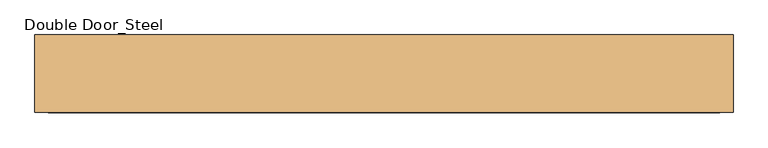
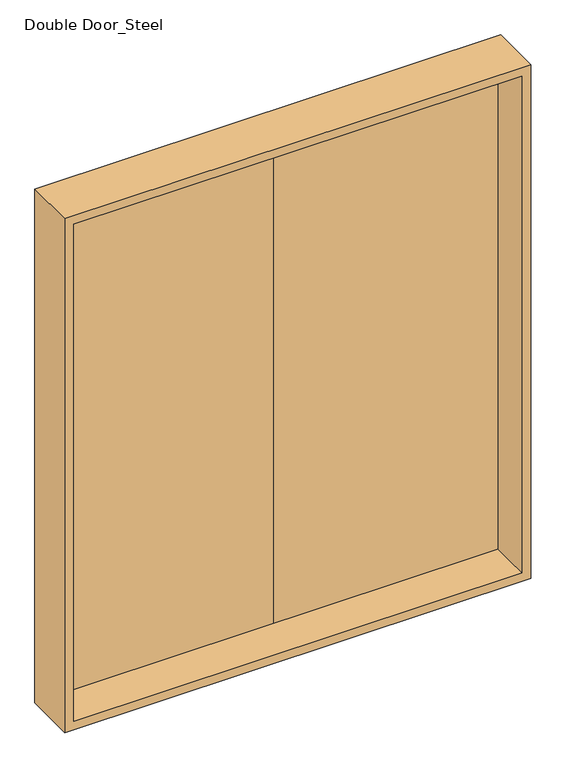
"""IFC4 building model written with IfcOpenShell, lengths in millimetres: door geometry, Double Door_Steel : H_DR_AR_B12_Double Door_Steel_W2000xH2100."""

import ifcopenshell
import ifcopenshell.guid

model = None  # the IFC model being written
_history = None  # IfcOwnerHistory: only IFC2X3 demands one
_inside = {}  # id of a spatial element -> (the spatial element, [elements in it])
_under = {}  # id of a project, library or spatial element -> (it, [spatial elements below it])
_declared = {}  # id of a project -> (the project, [libraries it declares])
_typed = {}  # id of a type object -> (the type object, [elements of that type])
_made_of = {}  # id of a material, layer set ... -> (it, [elements and type objects made of it])


def new_model(schema):
    """Start an empty IFC model of exactly this schema.

    Asked for "IFC4X3", IfcOpenShell would pick the latest addendum, in which some entities
    have other attributes; the version numbers below select the first issue.
    IFC2X3 requires an IfcOwnerHistory on every rooted entity: one is made here for all.
    """
    global model, _history
    if schema == "IFC4X3":
        model = ifcopenshell.file(schema_version=(4, 3, 0, 0))
    else:
        model = ifcopenshell.file(schema=schema)
    _inside.clear()
    _under.clear()
    _declared.clear()
    _typed.clear()
    _made_of.clear()
    _history = None
    if model.schema == "IFC2X3":
        org = make("IfcOrganization", Name="unknown")
        user = make(
            "IfcPersonAndOrganization",
            ThePerson=make("IfcPerson", FamilyName="unknown"),
            TheOrganization=org,
        )
        app = make(
            "IfcApplication",
            ApplicationDeveloper=org,
            Version="unknown",
            ApplicationFullName="unknown",
            ApplicationIdentifier="unknown",
        )
        _history = make(
            "IfcOwnerHistory",
            OwningUser=user,
            OwningApplication=app,
            ChangeAction="ADDED",
            CreationDate=0,
        )
    return model


def make(cls, **values):
    """One entity of the class cls with the attributes given. An attribute that is None is left unset."""
    return model.create_entity(
        cls, **{name: value for name, value in values.items() if value is not None}
    )


def rooted(cls, **values):
    """An entity with a GlobalId (a new one), such as an element, a storey or a relation."""
    return make(cls, GlobalId=ifcopenshell.guid.new(), OwnerHistory=_history, **values)


def si_unit(unit_type, name, prefix=None):
    """IfcSIUnit, for example si_unit("LENGTHUNIT", "METRE", prefix="MILLI")."""
    return make("IfcSIUnit", UnitType=unit_type, Prefix=prefix, Name=name)


def assignment(units):
    """IfcUnitAssignment: the units of a project."""
    return None if units is None else make("IfcUnitAssignment", Units=units)


def point(xyz):
    """IfcCartesianPoint."""
    return None if xyz is None else make("IfcCartesianPoint", Coordinates=xyz)


def direction(xyz):
    """IfcDirection."""
    return None if xyz is None else make("IfcDirection", DirectionRatios=xyz)


def frame(location, z_axis=None, x_axis=None):
    """IfcAxis2Placement3D, a coordinate frame: its origin and axes. An axis left out is left unset."""
    return make(
        "IfcAxis2Placement3D",
        Location=point(location),
        Axis=direction(z_axis),
        RefDirection=direction(x_axis),
    )


def origin():
    """The frame at (0, 0, 0) with its axes left unset."""
    return frame((0.0, 0.0, 0.0))


def place(relative_to, where):
    """IfcLocalPlacement: puts the frame where relative to a parent placement (None: the world)."""
    return make(
        "IfcLocalPlacement", PlacementRelTo=relative_to, RelativePlacement=where
    )


def context(
    kind, dimensions, precision=None, world=None, true_north=None, identifier=None
):
    """IfcGeometricRepresentationContext, for example the 3D "Model" context."""
    return make(
        "IfcGeometricRepresentationContext",
        ContextIdentifier=identifier,
        ContextType=kind,
        CoordinateSpaceDimension=dimensions,
        Precision=precision,
        WorldCoordinateSystem=world,
        TrueNorth=true_north,
    )


def project(units=None, contexts=None):
    """IfcProject with its units and contexts."""
    return rooted(
        "IfcProject",
        Name="project",
        RepresentationContexts=contexts,
        UnitsInContext=assignment(units),
    )


def spatial(cls, under=None, at=None, **own):
    """A site, building, storey or space (cls), placed at a placement, below another one or the project."""
    s = rooted(cls, ObjectPlacement=at, **own)
    if under is not None:
        _under.setdefault(under.id(), (under, []))[1].append(s)
    return s


def polyline(points):
    """IfcPolyline through the points."""
    return make("IfcPolyline", Points=[point(p) for p in points])


def outline(outer, holes=None, kind="AREA"):
    """IfcArbitraryClosedProfileDef: a profile drawn as a closed curve; with holes, ...WithVoids."""
    if holes is None:
        return make("IfcArbitraryClosedProfileDef", ProfileType=kind, OuterCurve=outer)
    return make(
        "IfcArbitraryProfileDefWithVoids",
        ProfileType=kind,
        OuterCurve=outer,
        InnerCurves=holes,
    )


def extrude(swept, where, along, depth):
    """IfcExtrudedAreaSolid: the profile swept, set in the frame where, extruded along a direction by depth."""
    return make(
        "IfcExtrudedAreaSolid",
        SweptArea=swept,
        Position=where,
        ExtrudedDirection=direction(along),
        Depth=depth,
    )


def faces_of(points, faces, orient=None, outer=None):
    """IfcFace entities. A face is a list of loops; a loop is a list of indices into points, from 0.

    orient and outer hold one flag for each loop. By default every Orientation is true, the
    first loop of a face is its IfcFaceOuterBound and the others are IfcFaceBound.
    """
    made = []
    for i, loops in enumerate(faces):
        bounds = []
        for j, loop in enumerate(loops):
            is_outer = j == 0 if outer is None else outer[i][j]
            bounds.append(
                make(
                    "IfcFaceOuterBound" if is_outer else "IfcFaceBound",
                    Bound=make("IfcPolyLoop", Polygon=[points[k] for k in loop]),
                    Orientation=True if orient is None else orient[i][j],
                )
            )
        made.append(make("IfcFace", Bounds=bounds))
    return made


def faceted_brep(points, faces, orient=None, outer=None, voids=None):
    """IfcFacetedBrep: a solid bounded by flat faces; with voids (closed shells), ...WithVoids."""
    shared = [point(p) for p in points]
    hull = make("IfcClosedShell", CfsFaces=faces_of(shared, faces, orient, outer))
    if voids is None:
        return make("IfcFacetedBrep", Outer=hull)
    return make(
        "IfcFacetedBrepWithVoids",
        Outer=hull,
        Voids=[
            make(cls, CfsFaces=faces_of(shared, fs, o, b)) for cls, fs, o, b in voids
        ],
    )


def shape(context_of_items, identifier, shape_type, items):
    """IfcShapeRepresentation: the items that make up one representation, for example the "Body"."""
    return make(
        "IfcShapeRepresentation",
        ContextOfItems=context_of_items,
        RepresentationIdentifier=identifier,
        RepresentationType=shape_type,
        Items=items,
    )


def source(mapping_origin, context_of_items, identifier, shape_type, items):
    """IfcRepresentationMap: a shape defined once, which mapped items show again and again."""
    return make(
        "IfcRepresentationMap",
        MappingOrigin=mapping_origin,
        MappedRepresentation=shape(context_of_items, identifier, shape_type, items),
    )


def transform(
    local_origin,
    x_axis=None,
    y_axis=None,
    z_axis=None,
    scale=None,
    scale2=None,
    scale3=None,
    uniform=True,
):
    """IfcCartesianTransformationOperator3D, or its non-uniform kind. x_axis, y_axis, z_axis: its Axis1, 2, 3."""
    if uniform:
        return make(
            "IfcCartesianTransformationOperator3D",
            Axis1=direction(x_axis),
            Axis2=direction(y_axis),
            LocalOrigin=point(local_origin),
            Scale=scale,
            Axis3=direction(z_axis),
        )
    return make(
        "IfcCartesianTransformationOperator3DnonUniform",
        Axis1=direction(x_axis),
        Axis2=direction(y_axis),
        LocalOrigin=point(local_origin),
        Scale=scale,
        Axis3=direction(z_axis),
        Scale2=scale2,
        Scale3=scale3,
    )


def mapped(mapping_source, mapping_target):
    """IfcMappedItem: shows the shape of a source again, moved by a transform."""
    return make(
        "IfcMappedItem", MappingSource=mapping_source, MappingTarget=mapping_target
    )


def made_of(thing, what):
    """Note that an element or type object is made of a material, layer set ...; save() writes the relation."""
    if what is not None:
        _made_of.setdefault(what.id(), (what, []))[1].append(thing)
    return thing


def element(
    cls,
    number,
    at=None,
    inside=None,
    cuts=None,
    type_object=None,
    material=None,
    context=None,
    identifier="Body",
    shape_type=None,
    held_by="IfcProductDefinitionShape",
    body=None,
    shapes=None,
    **own,
):
    """One element of the class cls, such as IfcWall. Its Tag is "e" and its number.

    at: its placement. inside: the storey or other place that contains it. cuts: it is an
    opening in that element (IfcRelVoidsElement). A single representation is given by context,
    identifier, shape_type and body (its items); several are given by shapes. held_by: the class
    of the entity that holds the representations. save() writes the other relations.
    """
    e = rooted(cls, Tag="e%d" % number, ObjectPlacement=at, **own)
    if body is not None:
        shapes = [shape(context, identifier, shape_type, body)]
    if shapes is not None:
        e.Representation = make(held_by, Representations=shapes)
    if inside is not None:
        _inside.setdefault(inside.id(), (inside, []))[1].append(e)
    if cuts is not None:
        rooted(
            "IfcRelVoidsElement", RelatingBuildingElement=cuts, RelatedOpeningElement=e
        )
    if type_object is not None:
        _typed.setdefault(type_object.id(), (type_object, []))[1].append(e)
    return made_of(e, material)


def aggregate(whole, parts):
    """IfcRelAggregates: a whole, such as a stair, and the parts it consists of."""
    return rooted("IfcRelAggregates", RelatingObject=whole, RelatedObjects=parts)


def save(model, path):
    """Write the relations noted so far, then the file.

    IfcRelAggregates (storeys below a building ...), IfcRelContainedInSpatialStructure (elements
    in a storey), IfcRelDefinesByType, IfcRelAssociatesMaterial and IfcRelDeclares: one each for
    every whole, place, type object, material and project.
    """
    for whole, parts in _under.values():
        aggregate(whole, parts)
    for where, things in _inside.values():
        rooted(
            "IfcRelContainedInSpatialStructure",
            RelatedElements=things,
            RelatingStructure=where,
        )
    for kind, things in _typed.values():
        rooted("IfcRelDefinesByType", RelatedObjects=things, RelatingType=kind)
    for what, things in _made_of.values():
        rooted("IfcRelAssociatesMaterial", RelatedObjects=things, RelatingMaterial=what)
    for by, libraries in _declared.values():
        rooted("IfcRelDeclares", RelatingContext=by, RelatedDefinitions=libraries)
    model.write(path)


def double_door_steel_22a565f0(model_context):
    return source(origin(), model_context, "Body", "SolidModel", [
        extrude(outline(polyline([(880.0, 60.0), (0.0, 60.0), (0.0, 100.0), (880.0, 100.0), (880.0, 60.0)])), frame((0.0, 0.0, 20.0), z_axis=(0.0, 0.0, 1.0), x_axis=(1.0, 0.0, 0.0)), (0.0, 0.0, 1.0), 2060.0),
        extrude(outline(polyline([(0.0, 60.0), (-880.0, 60.0), (-880.0, 100.0), (0.0, 100.0), (0.0, 60.0)])), frame((0.0, 0.0, 20.0), z_axis=(0.0, 0.0, 1.0), x_axis=(1.0, 0.0, 0.0)), (0.0, 0.0, 1.0), 2060.0),
        faceted_brep([(900.0, -100.0, 2100.0), (900.0, 100.0, 2100.0), (-900.0, 100.0, 2100.0), (-900.0, -100.0, 2100.0), (865.0, 60.0, 2065.0), (865.0, -100.0, 2065.0), (-865.0, -100.0, 2065.0), (-865.0, 60.0, 2065.0), (880.0, 100.0, 2080.0), (880.0, 60.0, 2080.0), (-880.0, 60.0, 2080.0), (-880.0, 100.0, 2080.0), (-900.0, 100.0, 0.0), (-900.0, -100.0, 0.0), (-865.0, -100.0, 35.0), (-865.0, 60.0, 35.0), (-880.0, 60.0, 20.0), (-880.0, 100.0, 20.0), (900.0, 100.0, 0.0), (880.0, 100.0, 20.0), (900.0, -100.0, 0.0), (865.0, -100.0, 35.0), (865.0, 60.0, 35.0), (880.0, 60.0, 20.0)], [[[0, 1, 2, 3]], [[4, 5, 6, 7]], [[8, 9, 10, 11]], [[3, 2, 12, 13]], [[7, 6, 14, 15]], [[11, 10, 16, 17]], [[18, 12, 2, 1], [8, 11, 17, 19]], [[13, 12, 18, 20]], [[0, 3, 13, 20], [21, 14, 6, 5]], [[15, 14, 21, 22]], [[23, 16, 10, 9], [4, 7, 15, 22]], [[17, 16, 23, 19]], [[20, 18, 1, 0]], [[22, 21, 5, 4]], [[19, 23, 9, 8]]]),
    ])


if __name__ == "__main__":
    model = new_model("IFC4")
    model_context = context("Model", 3, world=origin())
    ifc_project = project(units=[si_unit("LENGTHUNIT", "METRE", prefix="MILLI")], contexts=[model_context])
    site = spatial("IfcSite", under=ifc_project)
    building = spatial("IfcBuilding", under=site)
    placement = place(None, origin())
    double_door_steel_shape = double_door_steel_22a565f0(model_context)
    element("IfcDoor", 1, ObjectType="Double Door_Steel : H_DR_AR_B12_Double Door_Steel_W2000xH2100", at=placement, inside=building, context=model_context, shape_type="MappedRepresentation", body=[
        mapped(double_door_steel_shape, transform((0.0, 0.0, 0.0), x_axis=(1.0, 0.0, 0.0), y_axis=(0.0, 1.0, 0.0), z_axis=(0.0, 0.0, 1.0))),
    ])
    save(model, "model.ifc")

# Revit data of these elements
# Project information
#   H_Seismic Condition = "A as per ASCE 7-10"
#   H_Soil Condition = "C as per ASCE 7-10"
#   H_Basic Wind Speed = "58.3m/s ASCE7-10"
#   Building Name = "설퍼로딩컨트롤빌딩"
#   H_DS Project Code = "FAASA2302"
#   H_Project Abbreviation = "SACE2"
#   H_Project Division = "화공"
#   H_Project Finish = "2027-03-05"
#   H_Project Location = "Jafurah, Saudi Arabia"
#   H_Project Start = "2024-01-03"
#   H_Project Type = "EPC"
#   H_Smart Code = "FAASA2302"
#   Project Issue Date = "Issue Date"
#   Project Status = "Project Status"
#   Client Name = "Owner"
#   Project Address = "Enter address here"
#   Project Name = "자푸라2"
#   Project Number = "0001"
# Type "Double Door_Steel : H_DR_AR_B12_Double Door_Steel_W2000xH2100"
#   Type Mark = ""
#   프레임 = ""
#   철물 = ""
#   유리/마감 = ""
#   위치/개소 = ""
#   부호 = "1/SD"
#   문번호 = ""
#   문기호 = "SD"
#   Analytic Construction = "<None>"
#   Height = 2100 mm
#   Width = 1800 mm
#   Define Thermal Properties by = 1
#   문 틀 = none
#   문 = none
#   Function = (empty or 0)
#   Assembly Code = ""
#   Wall Closure = (empty or 0)
